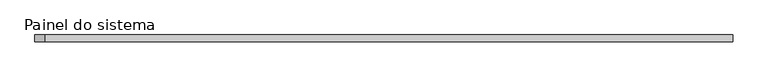
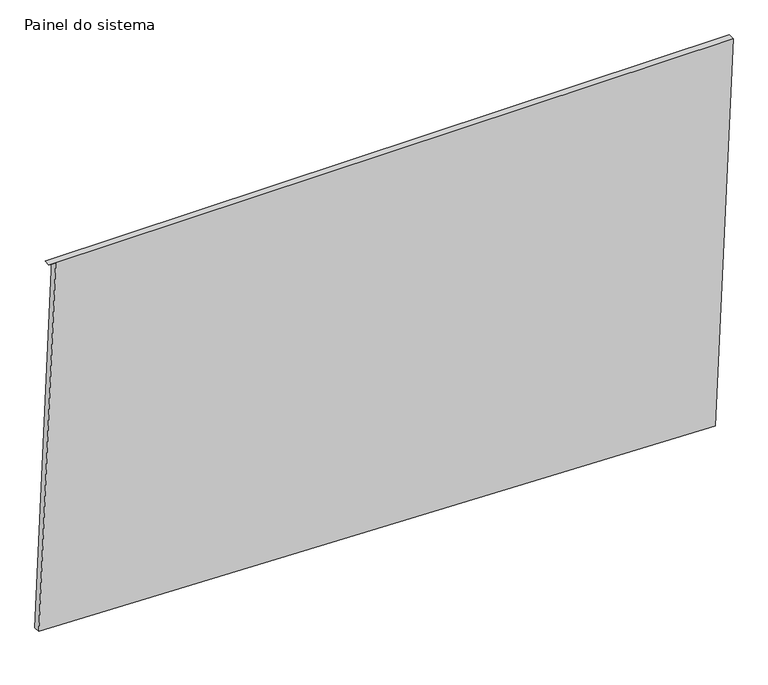
"""IFC4 building model written with IfcOpenShell, lengths in millimetres: plate geometry, Painel do sistema : Envidraçado."""

import ifcopenshell
import ifcopenshell.guid

model = None  # the IFC model being written
_history = None  # IfcOwnerHistory: only IFC2X3 demands one
_inside = {}  # id of a spatial element -> (the spatial element, [elements in it])
_under = {}  # id of a project, library or spatial element -> (it, [spatial elements below it])
_declared = {}  # id of a project -> (the project, [libraries it declares])
_typed = {}  # id of a type object -> (the type object, [elements of that type])
_made_of = {}  # id of a material, layer set ... -> (it, [elements and type objects made of it])


def new_model(schema):
    """Start an empty IFC model of exactly this schema.

    Asked for "IFC4X3", IfcOpenShell would pick the latest addendum, in which some entities
    have other attributes; the version numbers below select the first issue.
    IFC2X3 requires an IfcOwnerHistory on every rooted entity: one is made here for all.
    """
    global model, _history
    if schema == "IFC4X3":
        model = ifcopenshell.file(schema_version=(4, 3, 0, 0))
    else:
        model = ifcopenshell.file(schema=schema)
    _inside.clear()
    _under.clear()
    _declared.clear()
    _typed.clear()
    _made_of.clear()
    _history = None
    if model.schema == "IFC2X3":
        org = make("IfcOrganization", Name="unknown")
        user = make(
            "IfcPersonAndOrganization",
            ThePerson=make("IfcPerson", FamilyName="unknown"),
            TheOrganization=org,
        )
        app = make(
            "IfcApplication",
            ApplicationDeveloper=org,
            Version="unknown",
            ApplicationFullName="unknown",
            ApplicationIdentifier="unknown",
        )
        _history = make(
            "IfcOwnerHistory",
            OwningUser=user,
            OwningApplication=app,
            ChangeAction="ADDED",
            CreationDate=0,
        )
    return model


def make(cls, **values):
    """One entity of the class cls with the attributes given. An attribute that is None is left unset."""
    return model.create_entity(
        cls, **{name: value for name, value in values.items() if value is not None}
    )


def rooted(cls, **values):
    """An entity with a GlobalId (a new one), such as an element, a storey or a relation."""
    return make(cls, GlobalId=ifcopenshell.guid.new(), OwnerHistory=_history, **values)


def si_unit(unit_type, name, prefix=None):
    """IfcSIUnit, for example si_unit("LENGTHUNIT", "METRE", prefix="MILLI")."""
    return make("IfcSIUnit", UnitType=unit_type, Prefix=prefix, Name=name)


def assignment(units):
    """IfcUnitAssignment: the units of a project."""
    return None if units is None else make("IfcUnitAssignment", Units=units)


def point(xyz):
    """IfcCartesianPoint."""
    return None if xyz is None else make("IfcCartesianPoint", Coordinates=xyz)


def direction(xyz):
    """IfcDirection."""
    return None if xyz is None else make("IfcDirection", DirectionRatios=xyz)


def frame(location, z_axis=None, x_axis=None):
    """IfcAxis2Placement3D, a coordinate frame: its origin and axes. An axis left out is left unset."""
    return make(
        "IfcAxis2Placement3D",
        Location=point(location),
        Axis=direction(z_axis),
        RefDirection=direction(x_axis),
    )


def origin():
    """The frame at (0, 0, 0) with its axes left unset."""
    return frame((0.0, 0.0, 0.0))


def place(relative_to, where):
    """IfcLocalPlacement: puts the frame where relative to a parent placement (None: the world)."""
    return make(
        "IfcLocalPlacement", PlacementRelTo=relative_to, RelativePlacement=where
    )


def context(
    kind, dimensions, precision=None, world=None, true_north=None, identifier=None
):
    """IfcGeometricRepresentationContext, for example the 3D "Model" context."""
    return make(
        "IfcGeometricRepresentationContext",
        ContextIdentifier=identifier,
        ContextType=kind,
        CoordinateSpaceDimension=dimensions,
        Precision=precision,
        WorldCoordinateSystem=world,
        TrueNorth=true_north,
    )


def project(units=None, contexts=None):
    """IfcProject with its units and contexts."""
    return rooted(
        "IfcProject",
        Name="project",
        RepresentationContexts=contexts,
        UnitsInContext=assignment(units),
    )


def spatial(cls, under=None, at=None, **own):
    """A site, building, storey or space (cls), placed at a placement, below another one or the project."""
    s = rooted(cls, ObjectPlacement=at, **own)
    if under is not None:
        _under.setdefault(under.id(), (under, []))[1].append(s)
    return s


def polyline(points):
    """IfcPolyline through the points."""
    return make("IfcPolyline", Points=[point(p) for p in points])


def outline(outer, holes=None, kind="AREA"):
    """IfcArbitraryClosedProfileDef: a profile drawn as a closed curve; with holes, ...WithVoids."""
    if holes is None:
        return make("IfcArbitraryClosedProfileDef", ProfileType=kind, OuterCurve=outer)
    return make(
        "IfcArbitraryProfileDefWithVoids",
        ProfileType=kind,
        OuterCurve=outer,
        InnerCurves=holes,
    )


def extrude(swept, where, along, depth):
    """IfcExtrudedAreaSolid: the profile swept, set in the frame where, extruded along a direction by depth."""
    return make(
        "IfcExtrudedAreaSolid",
        SweptArea=swept,
        Position=where,
        ExtrudedDirection=direction(along),
        Depth=depth,
    )


def shape(context_of_items, identifier, shape_type, items):
    """IfcShapeRepresentation: the items that make up one representation, for example the "Body"."""
    return make(
        "IfcShapeRepresentation",
        ContextOfItems=context_of_items,
        RepresentationIdentifier=identifier,
        RepresentationType=shape_type,
        Items=items,
    )


def source(mapping_origin, context_of_items, identifier, shape_type, items):
    """IfcRepresentationMap: a shape defined once, which mapped items show again and again."""
    return make(
        "IfcRepresentationMap",
        MappingOrigin=mapping_origin,
        MappedRepresentation=shape(context_of_items, identifier, shape_type, items),
    )


def transform(
    local_origin,
    x_axis=None,
    y_axis=None,
    z_axis=None,
    scale=None,
    scale2=None,
    scale3=None,
    uniform=True,
):
    """IfcCartesianTransformationOperator3D, or its non-uniform kind. x_axis, y_axis, z_axis: its Axis1, 2, 3."""
    if uniform:
        return make(
            "IfcCartesianTransformationOperator3D",
            Axis1=direction(x_axis),
            Axis2=direction(y_axis),
            LocalOrigin=point(local_origin),
            Scale=scale,
            Axis3=direction(z_axis),
        )
    return make(
        "IfcCartesianTransformationOperator3DnonUniform",
        Axis1=direction(x_axis),
        Axis2=direction(y_axis),
        LocalOrigin=point(local_origin),
        Scale=scale,
        Axis3=direction(z_axis),
        Scale2=scale2,
        Scale3=scale3,
    )


def mapped(mapping_source, mapping_target):
    """IfcMappedItem: shows the shape of a source again, moved by a transform."""
    return make(
        "IfcMappedItem", MappingSource=mapping_source, MappingTarget=mapping_target
    )


def made_of(thing, what):
    """Note that an element or type object is made of a material, layer set ...; save() writes the relation."""
    if what is not None:
        _made_of.setdefault(what.id(), (what, []))[1].append(thing)
    return thing


def element(
    cls,
    number,
    at=None,
    inside=None,
    cuts=None,
    type_object=None,
    material=None,
    context=None,
    identifier="Body",
    shape_type=None,
    held_by="IfcProductDefinitionShape",
    body=None,
    shapes=None,
    **own,
):
    """One element of the class cls, such as IfcWall. Its Tag is "e" and its number.

    at: its placement. inside: the storey or other place that contains it. cuts: it is an
    opening in that element (IfcRelVoidsElement). A single representation is given by context,
    identifier, shape_type and body (its items); several are given by shapes. held_by: the class
    of the entity that holds the representations. save() writes the other relations.
    """
    e = rooted(cls, Tag="e%d" % number, ObjectPlacement=at, **own)
    if body is not None:
        shapes = [shape(context, identifier, shape_type, body)]
    if shapes is not None:
        e.Representation = make(held_by, Representations=shapes)
    if inside is not None:
        _inside.setdefault(inside.id(), (inside, []))[1].append(e)
    if cuts is not None:
        rooted(
            "IfcRelVoidsElement", RelatingBuildingElement=cuts, RelatedOpeningElement=e
        )
    if type_object is not None:
        _typed.setdefault(type_object.id(), (type_object, []))[1].append(e)
    return made_of(e, material)


def aggregate(whole, parts):
    """IfcRelAggregates: a whole, such as a stair, and the parts it consists of."""
    return rooted("IfcRelAggregates", RelatingObject=whole, RelatedObjects=parts)


def save(model, path):
    """Write the relations noted so far, then the file.

    IfcRelAggregates (storeys below a building ...), IfcRelContainedInSpatialStructure (elements
    in a storey), IfcRelDefinesByType, IfcRelAssociatesMaterial and IfcRelDeclares: one each for
    every whole, place, type object, material and project.
    """
    for whole, parts in _under.values():
        aggregate(whole, parts)
    for where, things in _inside.values():
        rooted(
            "IfcRelContainedInSpatialStructure",
            RelatedElements=things,
            RelatingStructure=where,
        )
    for kind, things in _typed.values():
        rooted("IfcRelDefinesByType", RelatedObjects=things, RelatingType=kind)
    for what, things in _made_of.values():
        rooted("IfcRelAssociatesMaterial", RelatedObjects=things, RelatingMaterial=what)
    for by, libraries in _declared.values():
        rooted("IfcRelDeclares", RelatingContext=by, RelatedDefinitions=libraries)
    model.write(path)


def painel_do_sistema_9efb096e(model_context):
    return source(origin(), model_context, "Body", "SweptSolid", [
        extrude(outline(polyline([(72.8211161, -1293.9735954), (0.0, 1227.8894811), (1504.1224514, 1293.9735954), (1504.1224514, -1256.1130181), (1503.0251268, -1231.1371121), (72.8211161, -1293.9735954)])), frame((0.0, 24.5, 0.0), z_axis=(0.0, 1.0, 0.0), x_axis=(0.0, 0.0, 1.0)), (0.0, 0.0, 1.0), 25.0),
    ])


if __name__ == "__main__":
    model = new_model("IFC4")
    model_context = context("Model", 3, world=origin())
    ifc_project = project(units=[si_unit("LENGTHUNIT", "METRE", prefix="MILLI")], contexts=[model_context])
    site = spatial("IfcSite", under=ifc_project)
    building = spatial("IfcBuilding", under=site)
    placement = place(None, origin())
    painel_do_sistema_shape = painel_do_sistema_9efb096e(model_context)
    element("IfcPlate", 1, ObjectType="Painel do sistema : Envidraçado", at=placement, inside=building, context=model_context, shape_type="MappedRepresentation", body=[
        mapped(painel_do_sistema_shape, transform((0.0, 0.0, 0.0), x_axis=(1.0, 0.0, 0.0), y_axis=(0.0, 1.0, 0.0), z_axis=(0.0, 0.0, 1.0))),
    ])
    save(model, "model.ifc")

# Revit data of these elements
# Type "Painel do sistema : Envidraçado"
#   Construction Type Id = "GSP4R"
#   Analytic Construction = "Vidraça única Pilkington 1/8 pol"
#   Visual Light Transmittance = 0.9
#   Solar Heat Gain Coefficient = 0.86
#   Heat Transfer Coefficient (U) = 6.7069 W/(m²·K)
# Element 1 (IfcPlate, "Painel do sistema : Envidraçado")
#   Materials on its faces: "Vidro"
# Materials
#   "Vidro": class "Vidro", colour RGB 0 128 192, transparency 0.9, Description = "Vidro de sílica", Cost = 0
